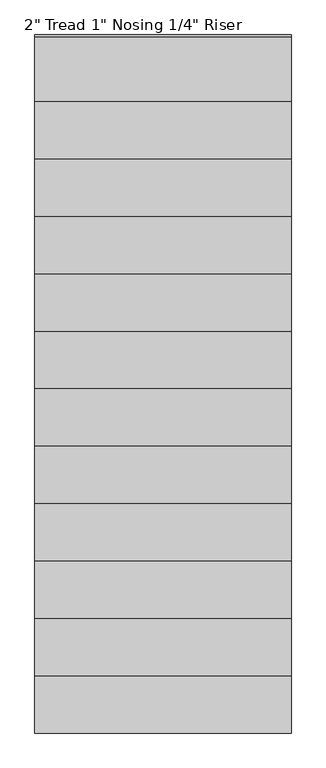
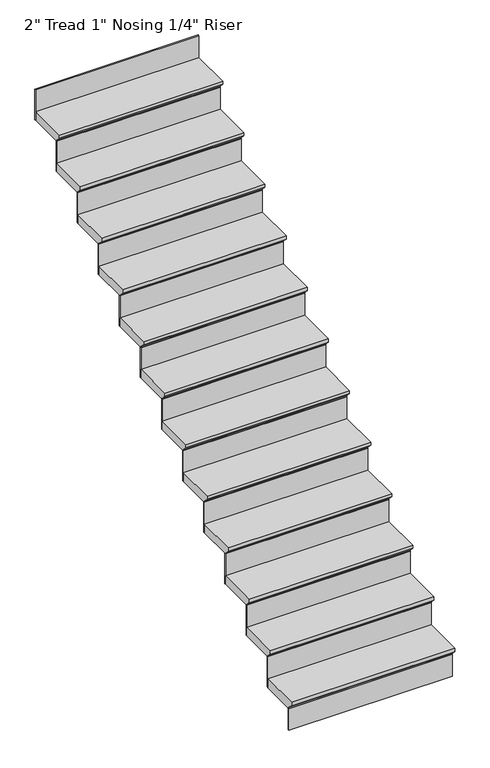
"""IFC4 building model written with IfcOpenShell, lengths in millimetres: stair flight geometry."""

import ifcopenshell
import ifcopenshell.guid

model = None  # the IFC model being written
_history = None  # IfcOwnerHistory: only IFC2X3 demands one
_inside = {}  # id of a spatial element -> (the spatial element, [elements in it])
_under = {}  # id of a project, library or spatial element -> (it, [spatial elements below it])
_declared = {}  # id of a project -> (the project, [libraries it declares])
_typed = {}  # id of a type object -> (the type object, [elements of that type])
_made_of = {}  # id of a material, layer set ... -> (it, [elements and type objects made of it])


def new_model(schema):
    """Start an empty IFC model of exactly this schema.

    Asked for "IFC4X3", IfcOpenShell would pick the latest addendum, in which some entities
    have other attributes; the version numbers below select the first issue.
    IFC2X3 requires an IfcOwnerHistory on every rooted entity: one is made here for all.
    """
    global model, _history
    if schema == "IFC4X3":
        model = ifcopenshell.file(schema_version=(4, 3, 0, 0))
    else:
        model = ifcopenshell.file(schema=schema)
    _inside.clear()
    _under.clear()
    _declared.clear()
    _typed.clear()
    _made_of.clear()
    _history = None
    if model.schema == "IFC2X3":
        org = make("IfcOrganization", Name="unknown")
        user = make(
            "IfcPersonAndOrganization",
            ThePerson=make("IfcPerson", FamilyName="unknown"),
            TheOrganization=org,
        )
        app = make(
            "IfcApplication",
            ApplicationDeveloper=org,
            Version="unknown",
            ApplicationFullName="unknown",
            ApplicationIdentifier="unknown",
        )
        _history = make(
            "IfcOwnerHistory",
            OwningUser=user,
            OwningApplication=app,
            ChangeAction="ADDED",
            CreationDate=0,
        )
    return model


def make(cls, **values):
    """One entity of the class cls with the attributes given. An attribute that is None is left unset."""
    return model.create_entity(
        cls, **{name: value for name, value in values.items() if value is not None}
    )


def rooted(cls, **values):
    """An entity with a GlobalId (a new one), such as an element, a storey or a relation."""
    return make(cls, GlobalId=ifcopenshell.guid.new(), OwnerHistory=_history, **values)


def si_unit(unit_type, name, prefix=None):
    """IfcSIUnit, for example si_unit("LENGTHUNIT", "METRE", prefix="MILLI")."""
    return make("IfcSIUnit", UnitType=unit_type, Prefix=prefix, Name=name)


def assignment(units):
    """IfcUnitAssignment: the units of a project."""
    return None if units is None else make("IfcUnitAssignment", Units=units)


def point(xyz):
    """IfcCartesianPoint."""
    return None if xyz is None else make("IfcCartesianPoint", Coordinates=xyz)


def direction(xyz):
    """IfcDirection."""
    return None if xyz is None else make("IfcDirection", DirectionRatios=xyz)


def frame(location, z_axis=None, x_axis=None):
    """IfcAxis2Placement3D, a coordinate frame: its origin and axes. An axis left out is left unset."""
    return make(
        "IfcAxis2Placement3D",
        Location=point(location),
        Axis=direction(z_axis),
        RefDirection=direction(x_axis),
    )


def origin():
    """The frame at (0, 0, 0) with its axes left unset."""
    return frame((0.0, 0.0, 0.0))


def place(relative_to, where):
    """IfcLocalPlacement: puts the frame where relative to a parent placement (None: the world)."""
    return make(
        "IfcLocalPlacement", PlacementRelTo=relative_to, RelativePlacement=where
    )


def context(
    kind, dimensions, precision=None, world=None, true_north=None, identifier=None
):
    """IfcGeometricRepresentationContext, for example the 3D "Model" context."""
    return make(
        "IfcGeometricRepresentationContext",
        ContextIdentifier=identifier,
        ContextType=kind,
        CoordinateSpaceDimension=dimensions,
        Precision=precision,
        WorldCoordinateSystem=world,
        TrueNorth=true_north,
    )


def project(units=None, contexts=None):
    """IfcProject with its units and contexts."""
    return rooted(
        "IfcProject",
        Name="project",
        RepresentationContexts=contexts,
        UnitsInContext=assignment(units),
    )


def spatial(cls, under=None, at=None, **own):
    """A site, building, storey or space (cls), placed at a placement, below another one or the project."""
    s = rooted(cls, ObjectPlacement=at, **own)
    if under is not None:
        _under.setdefault(under.id(), (under, []))[1].append(s)
    return s


def polyline(points):
    """IfcPolyline through the points."""
    return make("IfcPolyline", Points=[point(p) for p in points])


def outline(outer, holes=None, kind="AREA"):
    """IfcArbitraryClosedProfileDef: a profile drawn as a closed curve; with holes, ...WithVoids."""
    if holes is None:
        return make("IfcArbitraryClosedProfileDef", ProfileType=kind, OuterCurve=outer)
    return make(
        "IfcArbitraryProfileDefWithVoids",
        ProfileType=kind,
        OuterCurve=outer,
        InnerCurves=holes,
    )


def extrude(swept, where, along, depth):
    """IfcExtrudedAreaSolid: the profile swept, set in the frame where, extruded along a direction by depth."""
    return make(
        "IfcExtrudedAreaSolid",
        SweptArea=swept,
        Position=where,
        ExtrudedDirection=direction(along),
        Depth=depth,
    )


def shape(context_of_items, identifier, shape_type, items):
    """IfcShapeRepresentation: the items that make up one representation, for example the "Body"."""
    return make(
        "IfcShapeRepresentation",
        ContextOfItems=context_of_items,
        RepresentationIdentifier=identifier,
        RepresentationType=shape_type,
        Items=items,
    )


def source(mapping_origin, context_of_items, identifier, shape_type, items):
    """IfcRepresentationMap: a shape defined once, which mapped items show again and again."""
    return make(
        "IfcRepresentationMap",
        MappingOrigin=mapping_origin,
        MappedRepresentation=shape(context_of_items, identifier, shape_type, items),
    )


def transform(
    local_origin,
    x_axis=None,
    y_axis=None,
    z_axis=None,
    scale=None,
    scale2=None,
    scale3=None,
    uniform=True,
):
    """IfcCartesianTransformationOperator3D, or its non-uniform kind. x_axis, y_axis, z_axis: its Axis1, 2, 3."""
    if uniform:
        return make(
            "IfcCartesianTransformationOperator3D",
            Axis1=direction(x_axis),
            Axis2=direction(y_axis),
            LocalOrigin=point(local_origin),
            Scale=scale,
            Axis3=direction(z_axis),
        )
    return make(
        "IfcCartesianTransformationOperator3DnonUniform",
        Axis1=direction(x_axis),
        Axis2=direction(y_axis),
        LocalOrigin=point(local_origin),
        Scale=scale,
        Axis3=direction(z_axis),
        Scale2=scale2,
        Scale3=scale3,
    )


def mapped(mapping_source, mapping_target):
    """IfcMappedItem: shows the shape of a source again, moved by a transform."""
    return make(
        "IfcMappedItem", MappingSource=mapping_source, MappingTarget=mapping_target
    )


def made_of(thing, what):
    """Note that an element or type object is made of a material, layer set ...; save() writes the relation."""
    if what is not None:
        _made_of.setdefault(what.id(), (what, []))[1].append(thing)
    return thing


def element(
    cls,
    number,
    at=None,
    inside=None,
    cuts=None,
    type_object=None,
    material=None,
    context=None,
    identifier="Body",
    shape_type=None,
    held_by="IfcProductDefinitionShape",
    body=None,
    shapes=None,
    **own,
):
    """One element of the class cls, such as IfcWall. Its Tag is "e" and its number.

    at: its placement. inside: the storey or other place that contains it. cuts: it is an
    opening in that element (IfcRelVoidsElement). A single representation is given by context,
    identifier, shape_type and body (its items); several are given by shapes. held_by: the class
    of the entity that holds the representations. save() writes the other relations.
    """
    e = rooted(cls, Tag="e%d" % number, ObjectPlacement=at, **own)
    if body is not None:
        shapes = [shape(context, identifier, shape_type, body)]
    if shapes is not None:
        e.Representation = make(held_by, Representations=shapes)
    if inside is not None:
        _inside.setdefault(inside.id(), (inside, []))[1].append(e)
    if cuts is not None:
        rooted(
            "IfcRelVoidsElement", RelatingBuildingElement=cuts, RelatedOpeningElement=e
        )
    if type_object is not None:
        _typed.setdefault(type_object.id(), (type_object, []))[1].append(e)
    return made_of(e, material)


def aggregate(whole, parts):
    """IfcRelAggregates: a whole, such as a stair, and the parts it consists of."""
    return rooted("IfcRelAggregates", RelatingObject=whole, RelatedObjects=parts)


def save(model, path):
    """Write the relations noted so far, then the file.

    IfcRelAggregates (storeys below a building ...), IfcRelContainedInSpatialStructure (elements
    in a storey), IfcRelDefinesByType, IfcRelAssociatesMaterial and IfcRelDeclares: one each for
    every whole, place, type object, material and project.
    """
    for whole, parts in _under.values():
        aggregate(whole, parts)
    for where, things in _inside.values():
        rooted(
            "IfcRelContainedInSpatialStructure",
            RelatedElements=things,
            RelatingStructure=where,
        )
    for kind, things in _typed.values():
        rooted("IfcRelDefinesByType", RelatedObjects=things, RelatingType=kind)
    for what, things in _made_of.values():
        rooted("IfcRelAssociatesMaterial", RelatedObjects=things, RelatingMaterial=what)
    for by, libraries in _declared.values():
        rooted("IfcRelDeclares", RelatingContext=by, RelatedDefinitions=libraries)
    model.write(path)


def stair_flight_e5d7f74a(model_context):
    return source(origin(), model_context, "Body", "SweptSolid", [
        extrude(outline(polyline([(-12572.2570712, -2157.0461538), (-12343.6570712, -2157.0461538), (-12343.6570712, -2207.8461538), (-12546.8570712, -2207.8461538), (-12546.8570712, -2201.4961538), (-12572.2570712, -2176.0961538), (-12572.2570712, -2157.0461538)])), frame((-25042.4664763, 0.0, 0.0), z_axis=(1.0, 0.0, 0.0), x_axis=(0.0, 1.0, 0.0)), (0.0, 0.0, 1.0), 908.05),
        extrude(outline(polyline([(-24134.4164763, -12540.5070712), (-24134.4164763, -12546.8570712), (-25042.4664763, -12546.8570712), (-25042.4664763, -12540.5070712), (-24134.4164763, -12540.5070712)])), frame((0.0, 0.0, -2336.8), z_axis=(0.0, 0.0, 1.0), x_axis=(1.0, 0.0, 0.0)), (0.0, 0.0, 1.0), 128.9538462),
        extrude(outline(polyline([(-24134.4164763, -12337.3070712), (-24134.4164763, -12343.6570712), (-25042.4664763, -12343.6570712), (-25042.4664763, -12337.3070712), (-24134.4164763, -12337.3070712)])), frame((0.0, 0.0, -2207.8461538), z_axis=(0.0, 0.0, 1.0), x_axis=(1.0, 0.0, 0.0)), (0.0, 0.0, 1.0), 179.7538462),
        extrude(outline(polyline([(-12369.0570712, -1977.2923077), (-12140.4570712, -1977.2923077), (-12140.4570712, -2028.0923077), (-12343.6570712, -2028.0923077), (-12343.6570712, -2021.7423077), (-12369.0570712, -1996.3423077), (-12369.0570712, -1977.2923077)])), frame((-25042.4664763, 0.0, 0.0), z_axis=(1.0, 0.0, 0.0), x_axis=(0.0, 1.0, 0.0)), (0.0, 0.0, 1.0), 908.05),
        extrude(outline(polyline([(-24134.4164763, -12134.1070712), (-24134.4164763, -12140.4570712), (-25042.4664763, -12140.4570712), (-25042.4664763, -12134.1070712), (-24134.4164763, -12134.1070712)])), frame((0.0, 0.0, -2028.0923077), z_axis=(0.0, 0.0, 1.0), x_axis=(1.0, 0.0, 0.0)), (0.0, 0.0, 1.0), 179.7538462),
        extrude(outline(polyline([(-12165.8570712, -1797.5384615), (-11937.2570712, -1797.5384615), (-11937.2570712, -1848.3384615), (-12140.4570712, -1848.3384615), (-12140.4570712, -1841.9884615), (-12165.8570712, -1816.5884615), (-12165.8570712, -1797.5384615)])), frame((-25042.4664763, 0.0, 0.0), z_axis=(1.0, 0.0, 0.0), x_axis=(0.0, 1.0, 0.0)), (0.0, 0.0, 1.0), 908.05),
        extrude(outline(polyline([(-24134.4164763, -11930.9070712), (-24134.4164763, -11937.2570712), (-25042.4664763, -11937.2570712), (-25042.4664763, -11930.9070712), (-24134.4164763, -11930.9070712)])), frame((0.0, 0.0, -1848.3384615), z_axis=(0.0, 0.0, 1.0), x_axis=(1.0, 0.0, 0.0)), (0.0, 0.0, 1.0), 179.7538462),
        extrude(outline(polyline([(-11962.6570712, -1617.7846154), (-11734.0570712, -1617.7846154), (-11734.0570712, -1668.5846154), (-11937.2570712, -1668.5846154), (-11937.2570712, -1662.2346154), (-11962.6570712, -1636.8346154), (-11962.6570712, -1617.7846154)])), frame((-25042.4664763, 0.0, 0.0), z_axis=(1.0, 0.0, 0.0), x_axis=(0.0, 1.0, 0.0)), (0.0, 0.0, 1.0), 908.05),
        extrude(outline(polyline([(-24134.4164763, -11727.7070712), (-24134.4164763, -11734.0570712), (-25042.4664763, -11734.0570712), (-25042.4664763, -11727.7070712), (-24134.4164763, -11727.7070712)])), frame((0.0, 0.0, -1668.5846154), z_axis=(0.0, 0.0, 1.0), x_axis=(1.0, 0.0, 0.0)), (0.0, 0.0, 1.0), 179.7538462),
        extrude(outline(polyline([(-11759.4570712, -1438.0307692), (-11530.8570712, -1438.0307692), (-11530.8570712, -1488.8307692), (-11734.0570712, -1488.8307692), (-11734.0570712, -1482.4807692), (-11759.4570712, -1457.0807692), (-11759.4570712, -1438.0307692)])), frame((-25042.4664763, 0.0, 0.0), z_axis=(1.0, 0.0, 0.0), x_axis=(0.0, 1.0, 0.0)), (0.0, 0.0, 1.0), 908.05),
        extrude(outline(polyline([(-24134.4164763, -11524.5070712), (-24134.4164763, -11530.8570712), (-25042.4664763, -11530.8570712), (-25042.4664763, -11524.5070712), (-24134.4164763, -11524.5070712)])), frame((0.0, 0.0, -1488.8307692), z_axis=(0.0, 0.0, 1.0), x_axis=(1.0, 0.0, 0.0)), (0.0, 0.0, 1.0), 179.7538462),
        extrude(outline(polyline([(-11556.2570712, -1258.2769231), (-11327.6570712, -1258.2769231), (-11327.6570712, -1309.0769231), (-11530.8570712, -1309.0769231), (-11530.8570712, -1302.7269231), (-11556.2570712, -1277.3269231), (-11556.2570712, -1258.2769231)])), frame((-25042.4664763, 0.0, 0.0), z_axis=(1.0, 0.0, 0.0), x_axis=(0.0, 1.0, 0.0)), (0.0, 0.0, 1.0), 908.05),
        extrude(outline(polyline([(-24134.4164763, -11321.3070712), (-24134.4164763, -11327.6570712), (-25042.4664763, -11327.6570712), (-25042.4664763, -11321.3070712), (-24134.4164763, -11321.3070712)])), frame((0.0, 0.0, -1309.0769231), z_axis=(0.0, 0.0, 1.0), x_axis=(1.0, 0.0, 0.0)), (0.0, 0.0, 1.0), 179.7538462),
        extrude(outline(polyline([(-11353.0570712, -1078.5230769), (-11124.4570712, -1078.5230769), (-11124.4570712, -1129.3230769), (-11327.6570712, -1129.3230769), (-11327.6570712, -1122.9730769), (-11353.0570712, -1097.5730769), (-11353.0570712, -1078.5230769)])), frame((-25042.4664763, 0.0, 0.0), z_axis=(1.0, 0.0, 0.0), x_axis=(0.0, 1.0, 0.0)), (0.0, 0.0, 1.0), 908.05),
        extrude(outline(polyline([(-24134.4164763, -11118.1070712), (-24134.4164763, -11124.4570712), (-25042.4664763, -11124.4570712), (-25042.4664763, -11118.1070712), (-24134.4164763, -11118.1070712)])), frame((0.0, 0.0, -1129.3230769), z_axis=(0.0, 0.0, 1.0), x_axis=(1.0, 0.0, 0.0)), (0.0, 0.0, 1.0), 179.7538462),
        extrude(outline(polyline([(-11149.8570712, -898.7692308), (-10921.2570712, -898.7692308), (-10921.2570712, -949.5692308), (-11124.4570712, -949.5692308), (-11124.4570712, -943.2192308), (-11149.8570712, -917.8192308), (-11149.8570712, -898.7692308)])), frame((-25042.4664763, 0.0, 0.0), z_axis=(1.0, 0.0, 0.0), x_axis=(0.0, 1.0, 0.0)), (0.0, 0.0, 1.0), 908.05),
        extrude(outline(polyline([(-24134.4164763, -10914.9070712), (-24134.4164763, -10921.2570712), (-25042.4664763, -10921.2570712), (-25042.4664763, -10914.9070712), (-24134.4164763, -10914.9070712)])), frame((0.0, 0.0, -949.5692308), z_axis=(0.0, 0.0, 1.0), x_axis=(1.0, 0.0, 0.0)), (0.0, 0.0, 1.0), 179.7538462),
        extrude(outline(polyline([(-10946.6570712, -719.0153846), (-10718.0570712, -719.0153846), (-10718.0570712, -769.8153846), (-10921.2570712, -769.8153846), (-10921.2570712, -763.4653846), (-10946.6570712, -738.0653846), (-10946.6570712, -719.0153846)])), frame((-25042.4664763, 0.0, 0.0), z_axis=(1.0, 0.0, 0.0), x_axis=(0.0, 1.0, 0.0)), (0.0, 0.0, 1.0), 908.05),
        extrude(outline(polyline([(-24134.4164763, -10711.7070712), (-24134.4164763, -10718.0570712), (-25042.4664763, -10718.0570712), (-25042.4664763, -10711.7070712), (-24134.4164763, -10711.7070712)])), frame((0.0, 0.0, -769.8153846), z_axis=(0.0, 0.0, 1.0), x_axis=(1.0, 0.0, 0.0)), (0.0, 0.0, 1.0), 179.7538462),
        extrude(outline(polyline([(-10743.4570712, -539.2615385), (-10514.8570712, -539.2615385), (-10514.8570712, -590.0615385), (-10718.0570712, -590.0615385), (-10718.0570712, -583.7115385), (-10743.4570712, -558.3115385), (-10743.4570712, -539.2615385)])), frame((-25042.4664763, 0.0, 0.0), z_axis=(1.0, 0.0, 0.0), x_axis=(0.0, 1.0, 0.0)), (0.0, 0.0, 1.0), 908.05),
        extrude(outline(polyline([(-24134.4164763, -10508.5070712), (-24134.4164763, -10514.8570712), (-25042.4664763, -10514.8570712), (-25042.4664763, -10508.5070712), (-24134.4164763, -10508.5070712)])), frame((0.0, 0.0, -590.0615385), z_axis=(0.0, 0.0, 1.0), x_axis=(1.0, 0.0, 0.0)), (0.0, 0.0, 1.0), 179.7538462),
        extrude(outline(polyline([(-10540.2570712, -359.5076923), (-10311.6570712, -359.5076923), (-10311.6570712, -410.3076923), (-10514.8570712, -410.3076923), (-10514.8570712, -403.9576923), (-10540.2570712, -378.5576923), (-10540.2570712, -359.5076923)])), frame((-25042.4664763, 0.0, 0.0), z_axis=(1.0, 0.0, 0.0), x_axis=(0.0, 1.0, 0.0)), (0.0, 0.0, 1.0), 908.05),
        extrude(outline(polyline([(-24134.4164763, -10305.3070712), (-24134.4164763, -10311.6570712), (-25042.4664763, -10311.6570712), (-25042.4664763, -10305.3070712), (-24134.4164763, -10305.3070712)])), frame((0.0, 0.0, -410.3076923), z_axis=(0.0, 0.0, 1.0), x_axis=(1.0, 0.0, 0.0)), (0.0, 0.0, 1.0), 179.7538462),
        extrude(outline(polyline([(-24134.4164763, -10102.1070712), (-24134.4164763, -10108.4570712), (-25042.4664763, -10108.4570712), (-25042.4664763, -10102.1070712), (-24134.4164763, -10102.1070712)])), frame((0.0, 0.0, -230.5538462), z_axis=(0.0, 0.0, 1.0), x_axis=(1.0, 0.0, 0.0)), (0.0, 0.0, 1.0), 179.7538462),
        extrude(outline(polyline([(-10337.0570712, -179.7538462), (-10108.4570712, -179.7538462), (-10108.4570712, -230.5538462), (-10311.6570712, -230.5538462), (-10311.6570712, -224.2038462), (-10337.0570712, -198.8038462), (-10337.0570712, -179.7538462)])), frame((-25042.4664763, 0.0, 0.0), z_axis=(1.0, 0.0, 0.0), x_axis=(0.0, 1.0, 0.0)), (0.0, 0.0, 1.0), 908.05),
    ])


if __name__ == "__main__":
    model = new_model("IFC4")
    model_context = context("Model", 3, world=origin())
    ifc_project = project(units=[si_unit("LENGTHUNIT", "METRE", prefix="MILLI")], contexts=[model_context])
    site = spatial("IfcSite", under=ifc_project)
    building = spatial("IfcBuilding", under=site)
    placement = place(None, origin())
    stair_flight_shape = stair_flight_e5d7f74a(model_context)
    element("IfcStairFlight", 1, ObjectType="2\" Tread 1\" Nosing 1/4\" Riser", at=placement, inside=building, context=model_context, shape_type="MappedRepresentation", body=[
        mapped(stair_flight_shape, transform((0.0, 0.0, 0.0), x_axis=(1.0, 0.0, 0.0), y_axis=(0.0, 1.0, 0.0), z_axis=(0.0, 0.0, 1.0))),
    ])
    save(model, "model.ifc")
